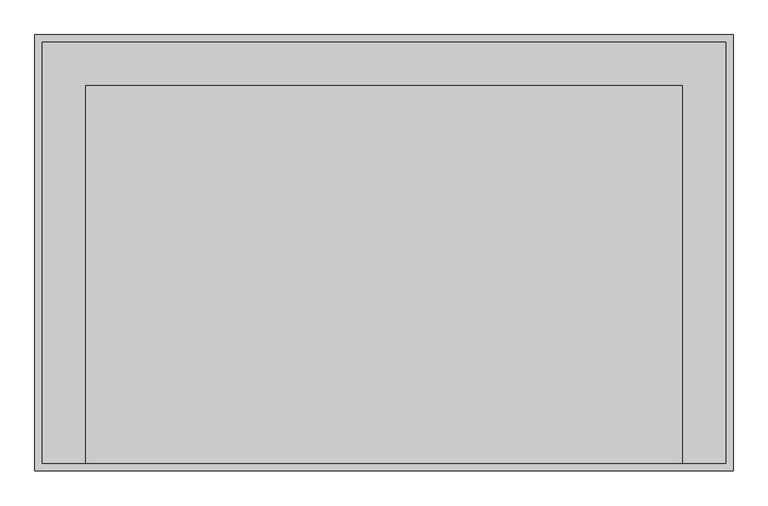
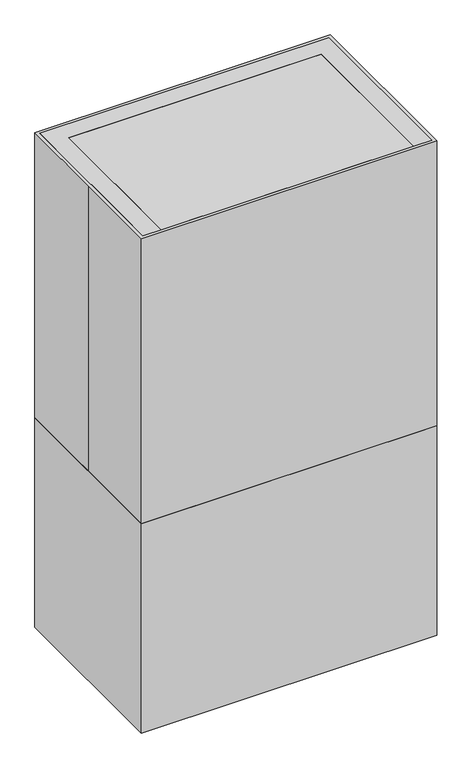
"""IFC4 building model written with IfcOpenShell, lengths in millimetres: proxy geometry, D0925 - Hood, Fume, Dental Acrylic, Floor Standing : D0925 - Hood, Fume, Dental Acrylic, Floor Standing."""

import ifcopenshell
import ifcopenshell.guid

model = None  # the IFC model being written
_history = None  # IfcOwnerHistory: only IFC2X3 demands one
_inside = {}  # id of a spatial element -> (the spatial element, [elements in it])
_under = {}  # id of a project, library or spatial element -> (it, [spatial elements below it])
_declared = {}  # id of a project -> (the project, [libraries it declares])
_typed = {}  # id of a type object -> (the type object, [elements of that type])
_made_of = {}  # id of a material, layer set ... -> (it, [elements and type objects made of it])


def new_model(schema):
    """Start an empty IFC model of exactly this schema.

    Asked for "IFC4X3", IfcOpenShell would pick the latest addendum, in which some entities
    have other attributes; the version numbers below select the first issue.
    IFC2X3 requires an IfcOwnerHistory on every rooted entity: one is made here for all.
    """
    global model, _history
    if schema == "IFC4X3":
        model = ifcopenshell.file(schema_version=(4, 3, 0, 0))
    else:
        model = ifcopenshell.file(schema=schema)
    _inside.clear()
    _under.clear()
    _declared.clear()
    _typed.clear()
    _made_of.clear()
    _history = None
    if model.schema == "IFC2X3":
        org = make("IfcOrganization", Name="unknown")
        user = make(
            "IfcPersonAndOrganization",
            ThePerson=make("IfcPerson", FamilyName="unknown"),
            TheOrganization=org,
        )
        app = make(
            "IfcApplication",
            ApplicationDeveloper=org,
            Version="unknown",
            ApplicationFullName="unknown",
            ApplicationIdentifier="unknown",
        )
        _history = make(
            "IfcOwnerHistory",
            OwningUser=user,
            OwningApplication=app,
            ChangeAction="ADDED",
            CreationDate=0,
        )
    return model


def make(cls, **values):
    """One entity of the class cls with the attributes given. An attribute that is None is left unset."""
    return model.create_entity(
        cls, **{name: value for name, value in values.items() if value is not None}
    )


def rooted(cls, **values):
    """An entity with a GlobalId (a new one), such as an element, a storey or a relation."""
    return make(cls, GlobalId=ifcopenshell.guid.new(), OwnerHistory=_history, **values)


def si_unit(unit_type, name, prefix=None):
    """IfcSIUnit, for example si_unit("LENGTHUNIT", "METRE", prefix="MILLI")."""
    return make("IfcSIUnit", UnitType=unit_type, Prefix=prefix, Name=name)


def assignment(units):
    """IfcUnitAssignment: the units of a project."""
    return None if units is None else make("IfcUnitAssignment", Units=units)


def point(xyz):
    """IfcCartesianPoint."""
    return None if xyz is None else make("IfcCartesianPoint", Coordinates=xyz)


def direction(xyz):
    """IfcDirection."""
    return None if xyz is None else make("IfcDirection", DirectionRatios=xyz)


def frame(location, z_axis=None, x_axis=None):
    """IfcAxis2Placement3D, a coordinate frame: its origin and axes. An axis left out is left unset."""
    return make(
        "IfcAxis2Placement3D",
        Location=point(location),
        Axis=direction(z_axis),
        RefDirection=direction(x_axis),
    )


def origin():
    """The frame at (0, 0, 0) with its axes left unset."""
    return frame((0.0, 0.0, 0.0))


def origin_with_axes():
    """The frame at (0, 0, 0) with the z axis (0, 0, 1) and the x axis (1, 0, 0) written out."""
    return frame((0.0, 0.0, 0.0), z_axis=(0.0, 0.0, 1.0), x_axis=(1.0, 0.0, 0.0))


def place(relative_to, where):
    """IfcLocalPlacement: puts the frame where relative to a parent placement (None: the world)."""
    return make(
        "IfcLocalPlacement", PlacementRelTo=relative_to, RelativePlacement=where
    )


def context(
    kind, dimensions, precision=None, world=None, true_north=None, identifier=None
):
    """IfcGeometricRepresentationContext, for example the 3D "Model" context."""
    return make(
        "IfcGeometricRepresentationContext",
        ContextIdentifier=identifier,
        ContextType=kind,
        CoordinateSpaceDimension=dimensions,
        Precision=precision,
        WorldCoordinateSystem=world,
        TrueNorth=true_north,
    )


def project(units=None, contexts=None):
    """IfcProject with its units and contexts."""
    return rooted(
        "IfcProject",
        Name="project",
        RepresentationContexts=contexts,
        UnitsInContext=assignment(units),
    )


def spatial(cls, under=None, at=None, **own):
    """A site, building, storey or space (cls), placed at a placement, below another one or the project."""
    s = rooted(cls, ObjectPlacement=at, **own)
    if under is not None:
        _under.setdefault(under.id(), (under, []))[1].append(s)
    return s


def polyline(points):
    """IfcPolyline through the points."""
    return make("IfcPolyline", Points=[point(p) for p in points])


def outline(outer, holes=None, kind="AREA"):
    """IfcArbitraryClosedProfileDef: a profile drawn as a closed curve; with holes, ...WithVoids."""
    if holes is None:
        return make("IfcArbitraryClosedProfileDef", ProfileType=kind, OuterCurve=outer)
    return make(
        "IfcArbitraryProfileDefWithVoids",
        ProfileType=kind,
        OuterCurve=outer,
        InnerCurves=holes,
    )


def extrude(swept, where, along, depth):
    """IfcExtrudedAreaSolid: the profile swept, set in the frame where, extruded along a direction by depth."""
    return make(
        "IfcExtrudedAreaSolid",
        SweptArea=swept,
        Position=where,
        ExtrudedDirection=direction(along),
        Depth=depth,
    )


def shape(context_of_items, identifier, shape_type, items):
    """IfcShapeRepresentation: the items that make up one representation, for example the "Body"."""
    return make(
        "IfcShapeRepresentation",
        ContextOfItems=context_of_items,
        RepresentationIdentifier=identifier,
        RepresentationType=shape_type,
        Items=items,
    )


def source(mapping_origin, context_of_items, identifier, shape_type, items):
    """IfcRepresentationMap: a shape defined once, which mapped items show again and again."""
    return make(
        "IfcRepresentationMap",
        MappingOrigin=mapping_origin,
        MappedRepresentation=shape(context_of_items, identifier, shape_type, items),
    )


def transform(
    local_origin,
    x_axis=None,
    y_axis=None,
    z_axis=None,
    scale=None,
    scale2=None,
    scale3=None,
    uniform=True,
):
    """IfcCartesianTransformationOperator3D, or its non-uniform kind. x_axis, y_axis, z_axis: its Axis1, 2, 3."""
    if uniform:
        return make(
            "IfcCartesianTransformationOperator3D",
            Axis1=direction(x_axis),
            Axis2=direction(y_axis),
            LocalOrigin=point(local_origin),
            Scale=scale,
            Axis3=direction(z_axis),
        )
    return make(
        "IfcCartesianTransformationOperator3DnonUniform",
        Axis1=direction(x_axis),
        Axis2=direction(y_axis),
        LocalOrigin=point(local_origin),
        Scale=scale,
        Axis3=direction(z_axis),
        Scale2=scale2,
        Scale3=scale3,
    )


def mapped(mapping_source, mapping_target):
    """IfcMappedItem: shows the shape of a source again, moved by a transform."""
    return make(
        "IfcMappedItem", MappingSource=mapping_source, MappingTarget=mapping_target
    )


def made_of(thing, what):
    """Note that an element or type object is made of a material, layer set ...; save() writes the relation."""
    if what is not None:
        _made_of.setdefault(what.id(), (what, []))[1].append(thing)
    return thing


def element(
    cls,
    number,
    at=None,
    inside=None,
    cuts=None,
    type_object=None,
    material=None,
    context=None,
    identifier="Body",
    shape_type=None,
    held_by="IfcProductDefinitionShape",
    body=None,
    shapes=None,
    **own,
):
    """One element of the class cls, such as IfcWall. Its Tag is "e" and its number.

    at: its placement. inside: the storey or other place that contains it. cuts: it is an
    opening in that element (IfcRelVoidsElement). A single representation is given by context,
    identifier, shape_type and body (its items); several are given by shapes. held_by: the class
    of the entity that holds the representations. save() writes the other relations.
    """
    e = rooted(cls, Tag="e%d" % number, ObjectPlacement=at, **own)
    if body is not None:
        shapes = [shape(context, identifier, shape_type, body)]
    if shapes is not None:
        e.Representation = make(held_by, Representations=shapes)
    if inside is not None:
        _inside.setdefault(inside.id(), (inside, []))[1].append(e)
    if cuts is not None:
        rooted(
            "IfcRelVoidsElement", RelatingBuildingElement=cuts, RelatedOpeningElement=e
        )
    if type_object is not None:
        _typed.setdefault(type_object.id(), (type_object, []))[1].append(e)
    return made_of(e, material)


def aggregate(whole, parts):
    """IfcRelAggregates: a whole, such as a stair, and the parts it consists of."""
    return rooted("IfcRelAggregates", RelatingObject=whole, RelatedObjects=parts)


def save(model, path):
    """Write the relations noted so far, then the file.

    IfcRelAggregates (storeys below a building ...), IfcRelContainedInSpatialStructure (elements
    in a storey), IfcRelDefinesByType, IfcRelAssociatesMaterial and IfcRelDeclares: one each for
    every whole, place, type object, material and project.
    """
    for whole, parts in _under.values():
        aggregate(whole, parts)
    for where, things in _inside.values():
        rooted(
            "IfcRelContainedInSpatialStructure",
            RelatedElements=things,
            RelatingStructure=where,
        )
    for kind, things in _typed.values():
        rooted("IfcRelDefinesByType", RelatedObjects=things, RelatingType=kind)
    for what, things in _made_of.values():
        rooted("IfcRelAssociatesMaterial", RelatedObjects=things, RelatingMaterial=what)
    for by, libraries in _declared.values():
        rooted("IfcRelDeclares", RelatingContext=by, RelatedDefinitions=libraries)
    model.write(path)


def specialty_equipment_1317bbbd(model_context):
    return source(origin(), model_context, "Body", "SweptSolid", [
        extrude(outline(polyline([(520.7, -368.3), (-520.7, -368.3), (-520.7, -342.9), (520.7, -342.9), (520.7, -368.3)])), frame((0.0, 0.0, 914.4), z_axis=(0.0, 0.0, 1.0), x_axis=(1.0, 0.0, 0.0)), (0.0, 0.0, 1.0), 762.0),
        extrude(outline(polyline([(520.7, -338.1852783), (-520.7, -338.1852783), (-520.7, 292.1), (520.7, 292.1), (520.7, -338.1852783)])), frame((0.0, 0.0, 1300.3613111), z_axis=(0.0, 0.0, 1.0), x_axis=(1.0, 0.0, 0.0)), (0.0, 0.0, 1.0), 12.7),
        extrude(outline(polyline([(520.7, -368.3), (-520.7, -368.3), (-520.7, 292.1), (520.7, 292.1), (520.7, -368.3)])), frame((0.0, 0.0, 1676.4), z_axis=(0.0, 0.0, 1.0), x_axis=(1.0, 0.0, 0.0)), (0.0, 0.0, 1.0), 482.6),
        extrude(outline(polyline([(-520.7, -368.3), (-596.9, -368.3), (-596.9, 368.3), (596.9, 368.3), (596.9, -368.3), (520.7, -368.3), (520.7, 292.1), (-520.7, 292.1), (-520.7, -368.3)])), frame((0.0, 0.0, 914.4), z_axis=(0.0, 0.0, 1.0), x_axis=(1.0, 0.0, 0.0)), (0.0, 0.0, 1.0), 1244.6),
        extrude(outline(polyline([(609.6, -381.0), (-609.6, -381.0), (-609.6, 381.0), (609.6, 381.0), (609.6, -381.0)])), origin_with_axes(), (0.0, 0.0, 1.0), 914.4),
        extrude(outline(polyline([(-609.6, 381.0), (609.6, 381.0), (609.6, -381.0), (-609.6, -381.0), (-609.6, 0.0), (-609.6, 381.0)])), origin_with_axes(), (0.0, 0.0, 1.0), 2159.0),
    ])


if __name__ == "__main__":
    model = new_model("IFC4")
    model_context = context("Model", 3, world=origin())
    ifc_project = project(units=[si_unit("LENGTHUNIT", "METRE", prefix="MILLI")], contexts=[model_context])
    site = spatial("IfcSite", under=ifc_project)
    building = spatial("IfcBuilding", under=site)
    placement = place(None, origin())
    specialty_equipment_shape = specialty_equipment_1317bbbd(model_context)
    element("IfcBuildingElementProxy", 1, Name="D0925 - Hood, Fume, Dental Acrylic, Floor Standing : D0925 - Hood, Fume, Dental Acrylic, Floor Standing", ObjectType="D0925 - Hood, Fume, Dental Acrylic, Floor Standing : D0925 - Hood, Fume, Dental Acrylic, Floor Standing", at=placement, inside=building, context=model_context, shape_type="MappedRepresentation", body=[
        mapped(specialty_equipment_shape, transform((0.0, 0.0, 0.0), x_axis=(1.0, 0.0, 0.0), y_axis=(0.0, 1.0, 0.0), z_axis=(0.0, 0.0, 1.0))),
    ])
    save(model, "model.ifc")

# Revit data of these elements
# Type "D0925 - Hood, Fume, Dental Acrylic, Floor Standing : D0925 - Hood, Fume, Dental Acrylic, Floor Standing"
#   Watts2 = "0"
#   Watts1 = "840"
#   Unit_Issue = "EA"
#   UTIL_6_Misc = "E"
#   UTIL_5_NonMedGas = "-"
#   UTIL_4_MiscGas = "-"
#   UTIL_3_MedGas = "-"
#   UTIL_2_Elec = "A"
#   UTIL_1_WaterDrain = "D"
#   Nomenclature = "Hood, Fume, Dental Acrylic, Floor Standing"
#   NSN = "6520"
#   Location [instance default] = ""
#   JSN = "D0925"
#   Fund_Source_VA = "-"
#   Fund_Source_Navy = "A"
#   Fund_Source_Army = "A"
#   Fund_Source_AF = "A"
#   ELEC_Volts2 = "0"
#   ELEC_Volts1 = "120"
#   ELEC_Phase2 = "0"
#   ELEC_Phase1 = "1"
#   ELEC_HertzSwitch = "0"
#   ELEC_HertzDependent = "-1"
#   ELEC_Hertz = "60"
#   ELEC_Amps2 = "0"
#   ELEC_Amps1 = "7"
#   DetailDescription = "Floor-standing fume hood workstation for processing acrylic dental resins. The fume hood is constructed of PVC plastic or other material resistant to acids and aggressive chemicals. The hood features built-in lighting, an extraction fan and a water channel for rinsing materials and containers. The hood has a counter-balanced vertically sliding front protective window."
#   CAT_VA = "A"
#   CAT_Navy = "A"
#   CAT_IHS = "-"
#   CAT_Army = "A"
#   CAT_AF = "A"
#   BTUperhour = "0"
#   Weight_IP = 570
#   DIM_Width_IP = 4' - 0"
#   DIM_Height_IP = 7' - 1"
#   DIM_Depth_IP = 2' - 6"
# Element 1 (IfcBuildingElementProxy, "D0925 - Hood, Fume, Dental Acrylic, Floor Standing : D0925 - Hood, Fume, Dental Acrylic, Floor Standing")
#   Materials on its faces: "EquipSpace", "Glass"
# Materials
#   "EquipSpace": class "Unassigned", colour RGB 221 217 195, transparency 0.5
#   "Glass": class "Glass", colour RGB 0 128 192, transparency 0.75
